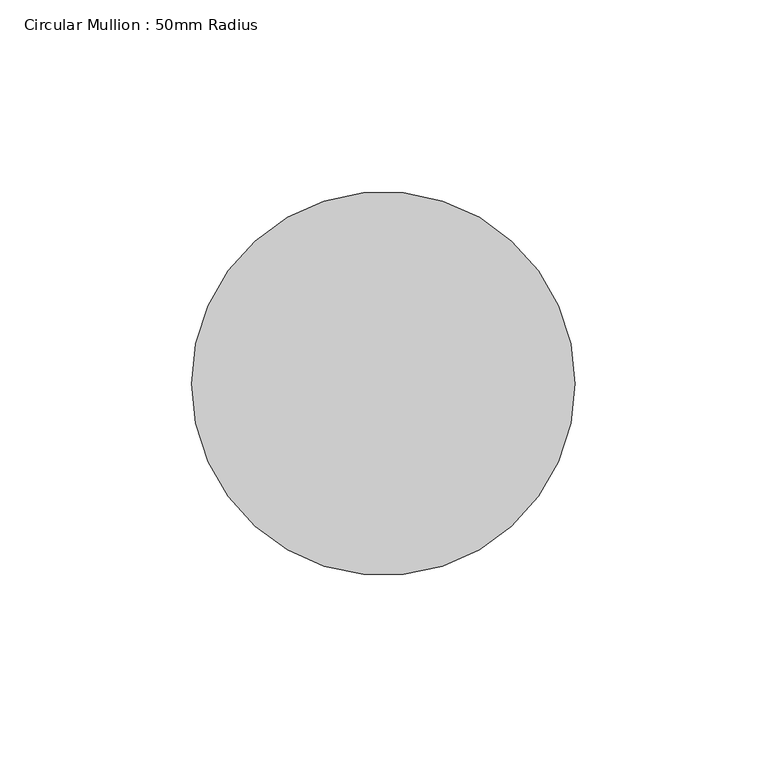
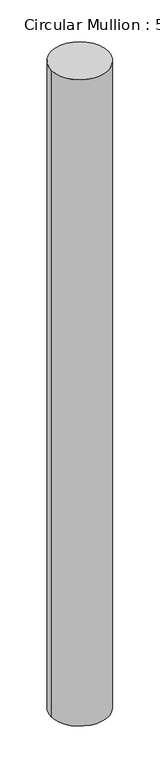
"""IFC4 building model written with IfcOpenShell, lengths in millimetres: member geometry, Circular Mullion : 50mm Radius."""

from ifc_helpers import new_model, si_unit, point, frame, origin, origin_2d, place, context, project, spatial, circle_curve, trimmed, segment, composite_curve, outline, extrude, source, transform, mapped, element, save


def circular_mullion_50mm_radius_16e3ce09(model_context):
    return source(origin(), model_context, "Body", "SweptSolid", [
        extrude(outline(composite_curve([segment(trimmed(circle_curve(origin_2d(), 50.0), [point((50.0, 0.0))], [point((-50.0, 0.0))], False, "CARTESIAN"), True, "CONTINUOUS"), segment(trimmed(circle_curve(origin_2d(), 50.0), [point((-50.0, 0.0))], [point((50.0, 0.0))], False, "CARTESIAN"), True, "CONTINUOUS")], self_intersect=False)), frame((0.0, 0.0, -1194.5252262), z_axis=(0.0, 0.0, 1.0), x_axis=(1.0, 0.0, 0.0)), (0.0, 0.0, 1.0), 1194.5252262),
    ])


if __name__ == "__main__":
    model = new_model("IFC4")
    model_context = context("Model", 3, world=origin())
    ifc_project = project(units=[si_unit("LENGTHUNIT", "METRE", prefix="MILLI")], contexts=[model_context])
    site = spatial("IfcSite", under=ifc_project)
    building = spatial("IfcBuilding", under=site)
    placement = place(None, origin())
    circular_mullion_50mm_radius_shape = circular_mullion_50mm_radius_16e3ce09(model_context)
    element("IfcMember", 1, ObjectType="Circular Mullion : 50mm Radius", at=placement, inside=building, context=model_context, shape_type="MappedRepresentation", body=[
        mapped(circular_mullion_50mm_radius_shape, transform((0.0, 0.0, 0.0), x_axis=(1.0, 0.0, 0.0), y_axis=(0.0, 1.0, 0.0), z_axis=(0.0, 0.0, 1.0))),
    ])
    save(model, "model.ifc")

# Revit data of these elements
# Type "Circular Mullion : 50mm Radius"
#   built-in parameter 1007350 = 0.164042 (stored number, unit not read)
# Element 1 (IfcMember, "Circular Mullion : 50mm Radius")
#   Materials on its faces: "Aluminium"
# Materials
#   "Aluminium": class "Metal", colour RGB 247 247 247, transparency 0, Description = "Aluminium 6061", Cost = 0
